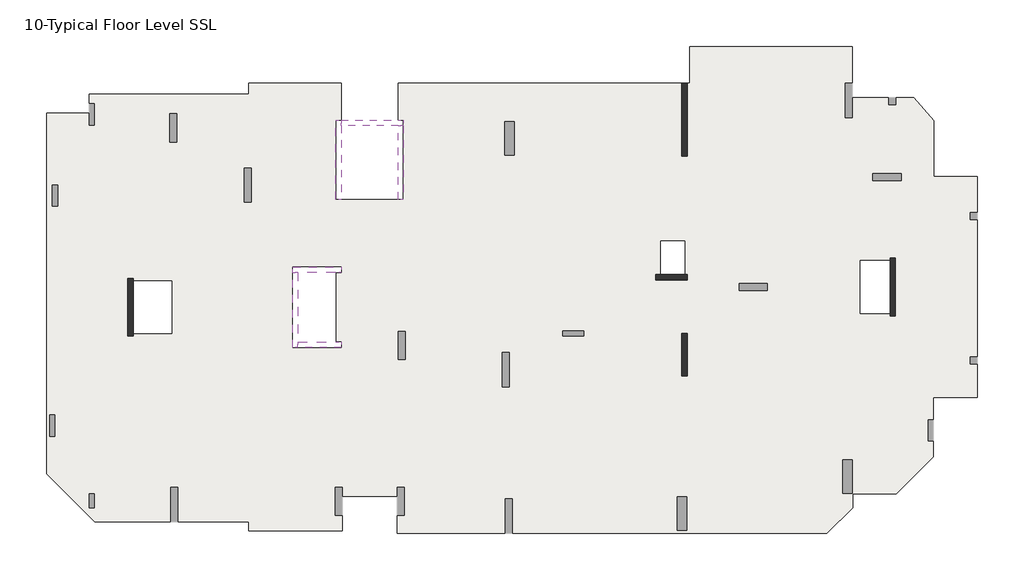
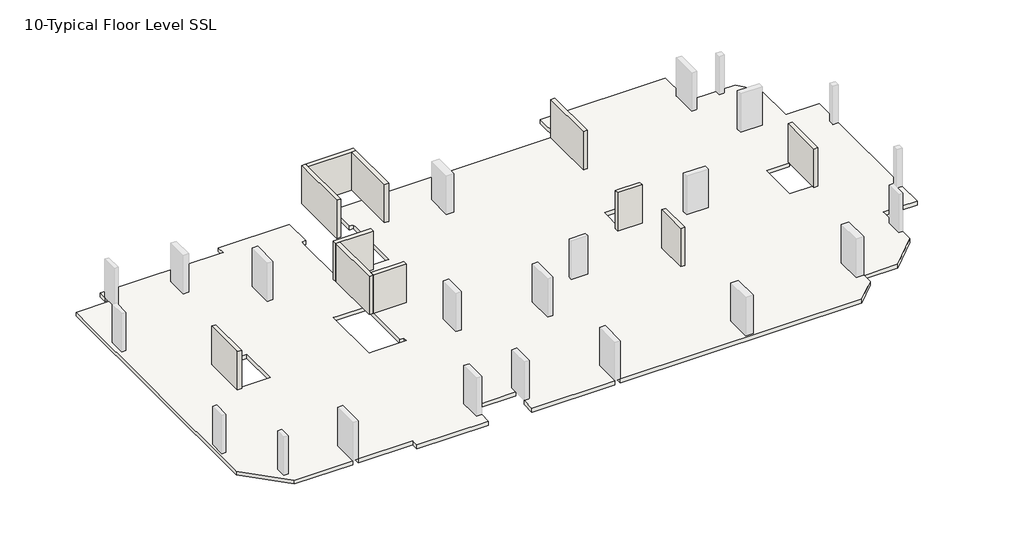
# One storey, part 1 of 2: 11 walls, 1 slab.
"""IFC4 building model written with IfcOpenShell, lengths in millimetres."""

from ifc_helpers import new_model, si_unit, origin, place, context, project, spatial, faceted_brep, element, save

model = new_model("IFC4")

# Units and contexts
model_context = context("Model", 3, world=origin())
ifc_project = project(units=[si_unit("LENGTHUNIT", "METRE", prefix="MILLI")], contexts=[model_context])

# Site, building, storey
site = spatial("IfcSite", under=ifc_project)
building = spatial("IfcBuilding", under=site)
storey = spatial("IfcBuildingStorey", under=building, Name="10-Typical Floor Level SSL", Elevation=24000.0)

# Slab
placement = place(None, origin())
element("IfcSlab", 1, ObjectType="Generic 300mm", at=placement, inside=storey, context=model_context, shape_type="Brep", body=[
    faceted_brep([(36192.0021644, 24072.000519, 23700.0), (36192.0021644, 26172.000519, 23700.0), (45446.0007483, 26172.000519, 23700.0), (45446.0007483, 24087.0, 23700.0), (45046.0007483, 24087.0, 23700.0), (45046.0007483, 22137.0, 23700.0), (45446.0007483, 22137.0, 23700.0), (45446.0007483, 23252.0000315, 23700.0), (47498.6337868, 23252.0000315, 23700.0), (47498.6337868, 22852.0, 23700.0), (47898.6337868, 22852.0, 23700.0), (47898.6337868, 23252.0000315, 23700.0), (48936.764334, 23252.0000315, 23700.0), (50076.0016214, 21956.8283806, 23700.0), (50076.0016214, 18780.0084406, 23700.0), (52549.9999998, 18780.0084406, 23700.0), (52549.9999998, 16712.0, 23700.0), (52149.9999998, 16712.0, 23700.0), (52149.9999998, 16312.0, 23700.0), (52549.9999998, 16312.0, 23700.0), (52549.9999998, 8504.0039609, 23700.0), (52149.9999998, 8504.0039609, 23700.0), (52149.9999998, 8104.0039609, 23700.0), (52549.9999998, 8104.0039609, 23700.0), (52549.9999998, 6204.0084406, 23700.0), (50046.0009271, 6204.0084406, 23700.0), (50046.0009271, 4931.9999929, 23700.0), (49746.0009271, 4931.9999929, 23700.0), (49746.0009271, 3731.9999929, 23700.0), (50046.0009271, 3731.9999929, 23700.0), (50046.0009271, 2810.5958657, 23700.0), (47943.4055804, 708.000519, 23700.0), (45456.0017287, 708.000519, 23700.0), (45456.0017287, -61.7051085, 23700.0), (43990.7023722, -1527.004465, 23700.0), (26113.9999998, -1527.004465, 23700.0), (26113.9999998, 422.995535, 23700.0), (25713.9999998, 422.995535, 23700.0), (25713.9999998, -1527.004465, 23700.0), (19569.9997488, -1527.004465, 23700.0), (19569.9997488, -512.0044652, 23700.0), (19969.9997488, -512.0044652, 23700.0), (19969.9997488, 1087.9955348, 23700.0), (19569.9997488, 1087.9955348, 23700.0), (19569.9997488, 564.000519, 23700.0), (16429.9999981, 564.000519, 23700.0), (16429.9999981, 1088.0, 23700.0), (16029.9999981, 1088.0, 23700.0), (16029.9999981, -512.0, 23700.0), (16429.9999981, -512.0, 23700.0), (16429.9999981, -1391.999481, 23700.0), (11136.0000923, -1391.999481, 23700.0), (11136.0000923, -866.9999847, 23700.0), (7082.0000416, -866.9999847, 23700.0), (7082.0000416, 1083.0000153, 23700.0), (6682.0000416, 1083.0000153, 23700.0), (6682.0000416, -866.9999847, 23700.0), (2364.4419097, -866.9999847, 23700.0), (-372.0, 1869.441925, 23700.0), (-372.0, 22380.0004589, 23700.0), (2052.0, 22380.0004589, 23700.0), (2052.0, 21708.0000656, 23700.0), (2352.0, 21708.0000656, 23700.0), (2352.0, 22908.0000656, 23700.0), (2052.0, 22908.0000656, 23700.0), (2052.0, 23472.000519, 23700.0), (11136.0000923, 23472.000519, 23700.0), (11136.0000923, 24072.000519, 23700.0), (16380.0000168, 24072.000519, 23700.0), (16380.0000168, 21972.0, 23700.0), (16079.9999997, 21972.0, 23700.0), (16079.9999997, 21672.0, 23700.0), (16079.9999997, 17468.0, 23700.0), (16379.9999997, 17468.0, 23700.0), (19619.9999997, 17468.0, 23700.0), (19919.9999997, 17468.0, 23700.0), (19919.9999997, 21672.0, 23700.0), (19919.9999997, 21972.0, 23700.0), (19619.9997365, 21972.0, 23700.0), (19619.9997365, 24072.000519, 23700.0), (35747.9999998, 24072.000519, 23700.0), (35747.9999998, 19932.0, 23700.0), (36047.9999998, 19932.0, 23700.0), (36047.9999998, 24072.000519, 23700.0), (16079.9999907, 9359.999998, 23700.0), (16079.9999907, 13320.0000002, 23700.0), (16380.0000168, 13320.0000002, 23700.0), (16380.0000168, 13620.0000002, 23700.0), (13919.9999907, 13620.0000002, 23700.0), (13619.9999907, 13620.0000002, 23700.0), (13619.9999907, 13320.0000002, 23700.0), (13619.9999907, 9359.999998, 23700.0), (13619.9999907, 9059.999998, 23700.0), (13919.9999907, 9059.999998, 23700.0), (16380.0000168, 9059.999998, 23700.0), (16380.0000168, 9359.999998, 23700.0), (4548.0000034, 9840.0000003, 23700.0), (6743.9999995, 9840.0000003, 23700.0), (6743.9999995, 12840.0000003, 23700.0), (4548.0000034, 12840.0000003, 23700.0), (4548.0000025, 12984.0000001, 23700.0), (4248.0000025, 12984.0000001, 23700.0), (4248.0000025, 9696.0, 23700.0), (4548.0000025, 9696.0, 23700.0), (47580.0014798, 13992.0079177, 23700.0), (45900.001729, 13992.0079177, 23700.0), (45900.001729, 10992.0079181, 23700.0), (47580.0014798, 10992.0079181, 23700.0), (47580.0014811, 10848.0079202, 23700.0), (47880.0014811, 10848.0079202, 23700.0), (47880.0014811, 14136.0000002, 23700.0), (47580.0014811, 14136.0000002, 23700.0), (35904.002157, 15108.0000083, 23700.0), (34548.0015145, 15108.0000083, 23700.0), (34548.0015145, 13199.9999992, 23700.0), (34248.0015201, 13199.9999992, 23700.0), (34248.0015201, 12899.9999992, 23700.0), (36048.0015201, 12899.9999992, 23700.0), (36048.0015201, 13199.9999992, 23700.0), (35904.002157, 13199.9999992, 23700.0), (257.9999999, 17088.0, 23700.0), (257.9999999, 18288.0, 23700.0), (-42.0000001, 18288.0, 23700.0), (-42.0000001, 17088.0, 23700.0), (108.001803, 4001.9999858, 23700.0), (108.001803, 5201.9999858, 23700.0), (-191.998197, 5201.9999858, 23700.0), (-191.998197, 4001.9999858, 23700.0), (30175.9999998, 9996.0000019, 23700.0), (28975.9999998, 9996.0000019, 23700.0), (28975.9999998, 9696.0000019, 23700.0), (30175.9999998, 9696.0000019, 23700.0), (7021.9999999, 20740.0000078, 23700.0), (7021.9999999, 22340.0000078, 23700.0), (6621.9999999, 22340.0000078, 23700.0), (6621.9999999, 20740.0000078, 23700.0), (48205.9993605, 18950.0, 23700.0), (46605.9993605, 18950.0, 23700.0), (46605.9993605, 18550.0, 23700.0), (48205.9993605, 18550.0, 23700.0), (20030.000009, 8355.9999979, 23700.0), (20030.000009, 9955.9999979, 23700.0), (19630.000009, 9955.9999979, 23700.0), (19630.000009, 8355.9999979, 23700.0), (11270.0000427, 17312.9999996, 23700.0), (11270.0000427, 19262.9999996, 23700.0), (10870.0000427, 19262.9999996, 23700.0), (10870.0000427, 17312.9999996, 23700.0), (40598.0014887, 12692.0079212, 23700.0), (38998.0014887, 12692.0079212, 23700.0), (38998.0014887, 12292.0079212, 23700.0), (40598.0014887, 12292.0079212, 23700.0), (2352.0, -72.0, 23700.0), (2352.0, 728.0, 23700.0), (2052.0, 728.0, 23700.0), (2052.0, -72.0, 23700.0), (25934.0000455, 6801.0001824, 23700.0), (25934.0000455, 8751.0001824, 23700.0), (25534.0000455, 8751.0001824, 23700.0), (25534.0000455, 6801.0001824, 23700.0), (36035.9999998, -1351.9992017, 23700.0), (36035.9999998, 548.0007983, 23700.0), (35485.9999998, 548.0007983, 23700.0), (35485.9999998, -1351.9992017, 23700.0), (45443.9999998, 748.0, 23700.0), (45443.9999998, 2648.0, 23700.0), (44893.9999998, 2648.0, 23700.0), (44893.9999998, 748.0, 23700.0), (26218.9999998, 20000.0, 23700.0), (26218.9999998, 21900.0, 23700.0), (25668.9999998, 21900.0, 23700.0), (25668.9999998, 20000.0, 23700.0), (35748.0054035, 9840.0000002, 23700.0), (35748.0054035, 7428.0000762, 23700.0), (36048.0054035, 7428.0000762, 23700.0), (36048.0054035, 9840.0000002, 23700.0), (36192.0021644, 26172.000519, 24000.0), (36192.0021644, 24072.000519, 24000.0), (36047.9999998, 24072.000519, 24000.0), (36047.9999998, 19932.0, 24000.0), (35747.9999998, 19932.0, 24000.0), (35747.9999998, 24072.000519, 24000.0), (19619.9997365, 24072.000519, 24000.0), (19619.9997365, 21972.0, 24000.0), (19919.9999997, 21972.0, 24000.0), (19919.9999997, 21672.0, 24000.0), (19919.9999997, 17468.0, 24000.0), (19619.9999997, 17468.0, 24000.0), (16379.9999997, 17468.0, 24000.0), (16079.9999997, 17468.0, 24000.0), (16079.9999997, 21672.0, 24000.0), (16079.9999997, 21972.0, 24000.0), (16380.0000168, 21972.0, 24000.0), (16380.0000168, 24072.000519, 24000.0), (11136.0000923, 24072.000519, 24000.0), (11136.0000923, 23472.000519, 24000.0), (2052.0, 23472.000519, 24000.0), (2052.0, 22908.0000656, 24000.0), (2352.0, 22908.0000656, 24000.0), (2352.0, 21708.0000656, 24000.0), (2052.0, 21708.0000656, 24000.0), (2052.0, 22380.0004589, 24000.0), (-372.0, 22380.0004589, 24000.0), (-372.0, 1869.441925, 24000.0), (2364.4419097, -866.9999847, 24000.0), (6682.0000416, -866.9999847, 24000.0), (6682.0000416, 1083.0000153, 24000.0), (7082.0000416, 1083.0000153, 24000.0), (7082.0000416, -866.9999847, 24000.0), (11136.0000923, -866.9999847, 24000.0), (11136.0000923, -1391.999481, 24000.0), (16429.9999981, -1391.999481, 24000.0), (16429.9999981, -512.0, 24000.0), (16029.9999981, -512.0, 24000.0), (16029.9999981, 1088.0, 24000.0), (16429.9999981, 1088.0, 24000.0), (16429.9999981, 564.000519, 24000.0), (19569.9997488, 564.000519, 24000.0), (19569.9997488, 1087.9955348, 24000.0), (19969.9997488, 1087.9955348, 24000.0), (19969.9997488, -512.0044652, 24000.0), (19569.9997488, -512.0044652, 24000.0), (19569.9997488, -1527.004465, 24000.0), (25713.9999998, -1527.004465, 24000.0), (25713.9999998, 422.995535, 24000.0), (26113.9999998, 422.995535, 24000.0), (26113.9999998, -1527.004465, 24000.0), (43990.7023722, -1527.004465, 24000.0), (45456.0017287, -61.7051085, 24000.0), (45456.0017287, 708.000519, 24000.0), (47943.4055804, 708.000519, 24000.0), (50046.0009271, 2810.5958657, 24000.0), (50046.0009271, 3731.9999929, 24000.0), (49746.0009271, 3731.9999929, 24000.0), (49746.0009271, 4931.9999929, 24000.0), (50046.0009271, 4931.9999929, 24000.0), (50046.0009271, 6204.0084406, 24000.0), (52549.9999998, 6204.0084406, 24000.0), (52549.9999998, 8104.0039609, 24000.0), (52149.9999998, 8104.0039609, 24000.0), (52149.9999998, 8504.0039609, 24000.0), (52549.9999998, 8504.0039609, 24000.0), (52549.9999998, 16312.0, 24000.0), (52149.9999998, 16312.0, 24000.0), (52149.9999998, 16712.0, 24000.0), (52549.9999998, 16712.0, 24000.0), (52549.9999998, 18780.0084406, 24000.0), (50076.0016214, 18780.0084406, 24000.0), (50076.0016214, 21956.8283806, 24000.0), (48936.764334, 23252.0000315, 24000.0), (47898.6337868, 23252.0000315, 24000.0), (47898.6337868, 22852.0, 24000.0), (47498.6337868, 22852.0, 24000.0), (47498.6337868, 23252.0000315, 24000.0), (45446.0006898, 23252.0000315, 24000.0), (45446.0007483, 22137.0, 24000.0), (45046.0007483, 22137.0, 24000.0), (45046.0007483, 24087.0, 24000.0), (45446.0007483, 24087.0, 24000.0), (45446.0007483, 26172.000519, 24000.0), (16079.9999907, 13320.0000002, 24000.0), (16079.9999907, 9359.999998, 24000.0), (16380.0000168, 9359.999998, 24000.0), (16380.0000168, 9059.999998, 24000.0), (13919.9999907, 9059.999998, 24000.0), (13619.9999907, 9059.999998, 24000.0), (13619.9999907, 9359.999998, 24000.0), (13619.9999907, 13320.0000002, 24000.0), (13619.9999907, 13620.0000002, 24000.0), (13919.9999907, 13620.0000002, 24000.0), (16380.0000168, 13620.0000002, 24000.0), (16380.0000168, 13320.0000002, 24000.0), (6743.9999995, 9840.0000003, 24000.0), (4548.0000034, 9840.0000003, 24000.0), (4548.0000025, 9696.0, 24000.0), (4248.0000025, 9696.0, 24000.0), (4248.0000025, 12984.0000001, 24000.0), (4548.0000025, 12984.0000001, 24000.0), (4548.0000025, 12840.0000003, 24000.0), (6743.9999995, 12840.0000003, 24000.0), (45900.001729, 13992.0079177, 24000.0), (47580.0014798, 13992.0079177, 24000.0), (47580.0014811, 14136.0000002, 24000.0), (47880.0014811, 14136.0000002, 24000.0), (47880.0014811, 10848.0079202, 24000.0), (47580.0014811, 10848.0079202, 24000.0), (47580.0014811, 10992.0079181, 24000.0), (45900.001729, 10992.0079181, 24000.0), (34548.0015145, 15108.0000083, 24000.0), (35904.002157, 15108.0000083, 24000.0), (35904.002157, 13199.9999992, 24000.0), (36048.0015201, 13199.9999992, 24000.0), (36048.0015201, 12899.9999992, 24000.0), (34248.0015201, 12899.9999992, 24000.0), (34248.0015201, 13199.9999992, 24000.0), (34548.0015145, 13199.9999992, 24000.0), (257.9999999, 18288.0, 24000.0), (257.9999999, 17088.0, 24000.0), (-42.0000001, 17088.0, 24000.0), (-42.0000001, 18288.0, 24000.0), (108.001803, 5201.9999858, 24000.0), (108.001803, 4001.9999858, 24000.0), (-191.998197, 4001.9999858, 24000.0), (-191.998197, 5201.9999858, 24000.0), (28975.9999998, 9996.0000019, 24000.0), (30175.9999998, 9996.0000019, 24000.0), (30175.9999998, 9696.0000019, 24000.0), (28975.9999998, 9696.0000019, 24000.0), (7021.9999999, 22340.0000078, 24000.0), (7021.9999999, 20740.0000078, 24000.0), (6621.9999999, 20740.0000078, 24000.0), (6621.9999999, 22340.0000078, 24000.0), (46605.9993605, 18950.0, 24000.0), (48205.9993605, 18950.0, 24000.0), (48205.9993605, 18550.0, 24000.0), (46605.9993605, 18550.0, 24000.0), (20030.000009, 9955.9999979, 24000.0), (20030.000009, 8355.9999979, 24000.0), (19630.000009, 8355.9999979, 24000.0), (19630.000009, 9955.9999979, 24000.0), (11270.0000427, 19262.9999996, 24000.0), (11270.0000427, 17312.9999996, 24000.0), (10870.0000427, 17312.9999996, 24000.0), (10870.0000427, 19262.9999996, 24000.0), (38998.0014887, 12692.0079212, 24000.0), (40598.0014887, 12692.0079212, 24000.0), (40598.0014887, 12292.0079212, 24000.0), (38998.0014887, 12292.0079212, 24000.0), (2352.0, 728.0, 24000.0), (2352.0, -72.0, 24000.0), (2052.0, -72.0, 24000.0), (2052.0, 728.0, 24000.0), (25934.0000455, 8751.0001824, 24000.0), (25934.0000455, 6801.0001824, 24000.0), (25534.0000455, 6801.0001824, 24000.0), (25534.0000455, 8751.0001824, 24000.0), (36035.9999998, 548.0007983, 24000.0), (36035.9999998, -1351.9992017, 24000.0), (35485.9999998, -1351.9992017, 24000.0), (35485.9999998, 548.0007983, 24000.0), (45443.9999998, 2648.0, 24000.0), (45443.9999998, 748.0, 24000.0), (44893.9999998, 748.0, 24000.0), (44893.9999998, 2648.0, 24000.0), (26218.9999998, 21900.0, 24000.0), (26218.9999998, 20000.0, 24000.0), (25668.9999998, 20000.0, 24000.0), (25668.9999998, 21900.0, 24000.0), (35748.0054035, 7428.0000762, 24000.0), (35748.0054035, 9840.0000002, 24000.0), (36048.0054035, 9840.0000002, 24000.0), (36048.0054035, 7428.0000762, 24000.0)], [[[0, 1, 2, 3, 4, 5, 6, 7, 8, 9, 10, 11, 12, 13, 14, 15, 16, 17, 18, 19, 20, 21, 22, 23, 24, 25, 26, 27, 28, 29, 30, 31, 32, 33, 34, 35, 36, 37, 38, 39, 40, 41, 42, 43, 44, 45, 46, 47, 48, 49, 50, 51, 52, 53, 54, 55, 56, 57, 58, 59, 60, 61, 62, 63, 64, 65, 66, 67, 68, 69, 70, 71, 72, 73, 74, 75, 76, 77, 78, 79, 80, 81, 82, 83], [84, 85, 86, 87, 88, 89, 90, 91, 92, 93, 94, 95], [96, 97, 98, 99, 100, 101, 102, 103], [104, 105, 106, 107, 108, 109, 110, 111], [112, 113, 114, 115, 116, 117, 118, 119], [120, 121, 122, 123], [124, 125, 126, 127], [128, 129, 130, 131], [132, 133, 134, 135], [136, 137, 138, 139], [140, 141, 142, 143], [144, 145, 146, 147], [148, 149, 150, 151], [152, 153, 154, 155], [156, 157, 158, 159], [160, 161, 162, 163], [164, 165, 166, 167], [168, 169, 170, 171], [172, 173, 174, 175]], [[176, 177, 178, 179, 180, 181, 182, 183, 184, 185, 186, 187, 188, 189, 190, 191, 192, 193, 194, 195, 196, 197, 198, 199, 200, 201, 202, 203, 204, 205, 206, 207, 208, 209, 210, 211, 212, 213, 214, 215, 216, 217, 218, 219, 220, 221, 222, 223, 224, 225, 226, 227, 228, 229, 230, 231, 232, 233, 234, 235, 236, 237, 238, 239, 240, 241, 242, 243, 244, 245, 246, 247, 248, 249, 250, 251, 252, 253, 254, 255, 256, 257, 258, 259], [260, 261, 262, 263, 264, 265, 266, 267, 268, 269, 270, 271], [272, 273, 274, 275, 276, 277, 278, 279], [280, 281, 282, 283, 284, 285, 286, 287], [288, 289, 290, 291, 292, 293, 294, 295], [296, 297, 298, 299], [300, 301, 302, 303], [304, 305, 306, 307], [308, 309, 310, 311], [312, 313, 314, 315], [316, 317, 318, 319], [320, 321, 322, 323], [324, 325, 326, 327], [328, 329, 330, 331], [332, 333, 334, 335], [336, 337, 338, 339], [340, 341, 342, 343], [344, 345, 346, 347], [348, 349, 350, 351]], [[68, 193, 192, 69]], [[182, 79, 78, 183]], [[79, 182, 181, 80]], [[177, 0, 83, 178]], [[1, 0, 177, 176]], [[2, 1, 176, 259]], [[3, 2, 259, 258]], [[249, 12, 11, 250]], [[7, 254, 253, 8]], [[13, 12, 249, 248]], [[14, 13, 248, 247]], [[15, 14, 247, 246]], [[15, 246, 245, 16]], [[237, 24, 23, 238]], [[19, 242, 241, 20]], [[25, 24, 237, 236]], [[25, 236, 235, 26]], [[231, 30, 29, 232]], [[32, 31, 230, 229]], [[33, 32, 229, 228]], [[34, 33, 228, 227]], [[34, 227, 226, 35]], [[222, 39, 38, 223]], [[39, 222, 221, 40]], [[45, 44, 217, 216]], [[211, 50, 49, 212]], [[51, 50, 211, 210]], [[52, 51, 210, 209]], [[52, 209, 208, 53]], [[204, 57, 56, 205]], [[58, 57, 204, 203]], [[59, 58, 203, 202]], [[60, 59, 202, 201]], [[196, 65, 64, 197]], [[66, 65, 196, 195]], [[67, 66, 195, 194]], [[68, 67, 194, 193]], [[31, 30, 231, 230]], [[85, 84, 261, 260]], [[72, 189, 188, 187, 186, 75, 74, 73]], [[272, 97, 96, 273]], [[97, 272, 279, 98]], [[98, 279, 278, 99]], [[280, 105, 104, 281]], [[105, 280, 287, 106]], [[106, 287, 286, 107]], [[112, 289, 288, 113]], [[113, 288, 295, 114]], [[289, 112, 119, 290]], [[62, 199, 198, 63]], [[199, 62, 61, 200]], [[200, 61, 60, 201]], [[63, 198, 197, 64]], [[120, 297, 296, 121]], [[297, 120, 123, 298]], [[298, 123, 122, 299]], [[299, 122, 121, 296]], [[124, 301, 300, 125]], [[301, 124, 127, 302]], [[302, 127, 126, 303]], [[303, 126, 125, 300]], [[28, 233, 232, 29]], [[233, 28, 27, 234]], [[234, 27, 26, 235]], [[128, 305, 304, 129]], [[305, 128, 131, 306]], [[306, 131, 130, 307]], [[307, 130, 129, 304]], [[132, 309, 308, 133]], [[309, 132, 135, 310]], [[310, 135, 134, 311]], [[311, 134, 133, 308]], [[41, 220, 219, 42]], [[220, 41, 40, 221]], [[43, 218, 217, 44]], [[218, 43, 42, 219]], [[136, 313, 312, 137]], [[313, 136, 139, 314]], [[314, 139, 138, 315]], [[315, 138, 137, 312]], [[140, 317, 316, 141]], [[317, 140, 143, 318]], [[318, 143, 142, 319]], [[319, 142, 141, 316]], [[215, 46, 45, 216]], [[48, 213, 212, 49]], [[213, 48, 47, 214]], [[214, 47, 46, 215]], [[144, 321, 320, 145]], [[321, 144, 147, 322]], [[322, 147, 146, 323]], [[323, 146, 145, 320]], [[207, 54, 53, 208]], [[55, 206, 205, 56]], [[206, 55, 54, 207]], [[225, 36, 35, 226]], [[37, 224, 223, 38]], [[224, 37, 36, 225]], [[6, 255, 254, 7]], [[255, 6, 5, 256]], [[256, 5, 4, 257]], [[257, 4, 3, 258]], [[148, 325, 324, 149]], [[325, 148, 151, 326]], [[326, 151, 150, 327]], [[327, 150, 149, 324]], [[152, 329, 328, 153]], [[329, 152, 155, 330]], [[330, 155, 154, 331]], [[331, 154, 153, 328]], [[156, 333, 332, 157]], [[333, 156, 159, 334]], [[334, 159, 158, 335]], [[335, 158, 157, 332]], [[160, 337, 336, 161]], [[337, 160, 163, 338]], [[338, 163, 162, 339]], [[339, 162, 161, 336]], [[164, 341, 340, 165]], [[341, 164, 167, 342]], [[342, 167, 166, 343]], [[343, 166, 165, 340]], [[168, 345, 344, 169]], [[345, 168, 171, 346]], [[346, 171, 170, 347]], [[347, 170, 169, 344]], [[70, 191, 190, 189, 72, 71]], [[191, 70, 69, 192]], [[77, 184, 183, 78]], [[184, 77, 76, 75, 186, 185]], [[271, 86, 85, 260]], [[87, 270, 269, 268, 89, 88]], [[86, 271, 270, 87]], [[89, 268, 267, 266, 265, 92, 91, 90]], [[92, 265, 264, 263, 94, 93]], [[95, 262, 261, 84]], [[262, 95, 94, 263]], [[277, 100, 99, 278]], [[103, 274, 273, 96]], [[101, 276, 275, 102]], [[100, 277, 276, 101]], [[274, 103, 102, 275]], [[116, 293, 292, 117]], [[118, 291, 290, 119]], [[294, 115, 114, 295]], [[117, 292, 291, 118]], [[293, 116, 115, 294]], [[172, 349, 348, 173]], [[174, 351, 350, 175]], [[173, 348, 351, 174]], [[349, 172, 175, 350]], [[285, 108, 107, 286]], [[111, 282, 281, 104]], [[109, 284, 283, 110]], [[108, 285, 284, 109]], [[282, 111, 110, 283]], [[82, 179, 178, 83]], [[180, 81, 80, 181]], [[179, 82, 81, 180]], [[18, 243, 242, 19]], [[243, 18, 17, 244]], [[244, 17, 16, 245]], [[10, 251, 250, 11]], [[251, 10, 9, 252]], [[252, 9, 8, 253]], [[22, 239, 238, 23]], [[239, 22, 21, 240]], [[240, 21, 20, 241]]]),
])

# Walls
element("IfcWall", 2, ObjectType="Shear Walls 300mm", at=placement, inside=storey, context=model_context, shape_type="Brep", body=[
    faceted_brep([(4548.0000025, 9696.0, 24000.0), (4548.0000025, 12984.0000001, 24000.0), (4548.0000025, 12984.0000001, 26700.0), (4548.0000025, 12984.0000001, 27000.0), (4548.0000025, 12840.0000003, 27000.0), (4548.0000025, 9840.0000003, 27000.0), (4548.0000025, 9696.0, 27000.0), (4548.0000025, 9696.0, 26700.0), (4248.0000025, 9696.0, 24000.0), (4248.0000025, 9696.0, 26700.0), (4248.0000025, 9696.0, 27000.0), (4248.0000025, 12984.0000001, 27000.0), (4248.0000025, 12984.0000001, 26700.0), (4248.0000025, 12984.0000001, 24000.0)], [[[0, 1, 2, 3, 4, 5, 6, 7]], [[8, 9, 10, 11, 12, 13]], [[1, 0, 8, 13]], [[3, 2, 1, 13, 12, 11]], [[6, 5, 4, 3, 11, 10]], [[0, 7, 6, 10, 9, 8]]]),
])
element("IfcWall", 3, ObjectType="Shear Walls 300mm", at=placement, inside=storey, context=model_context, shape_type="Brep", body=[
    faceted_brep([(34248.0015201, 12899.9999992, 24000.0), (36048.0015201, 12899.9999992, 24000.0), (36048.0015201, 12899.9999992, 26700.0), (36048.0015201, 12899.9999992, 27000.0), (34248.0015201, 12899.9999992, 27000.0), (34248.0015201, 12899.9999992, 26700.0), (34248.0015201, 13199.9999992, 24000.0), (34248.0015201, 13199.9999992, 26700.0), (34248.0015201, 13199.9999992, 27000.0), (34548.0015145, 13199.9999992, 27000.0), (35904.002157, 13199.9999992, 27000.0), (36048.0015201, 13199.9999992, 27000.0), (36048.0015201, 13199.9999992, 26700.0), (36048.0015201, 13199.9999992, 24000.0)], [[[0, 1, 2, 3, 4, 5]], [[6, 7, 8, 9, 10, 11, 12, 13]], [[1, 0, 6, 13]], [[3, 2, 1, 13, 12, 11]], [[4, 3, 11, 10, 9, 8]], [[0, 5, 4, 8, 7, 6]]]),
])
element("IfcWall", 4, ObjectType="Shear Walls 300mm", at=placement, inside=storey, context=model_context, shape_type="Brep", body=[
    faceted_brep([(35748.0054035, 9840.0000002, 24000.0), (35748.0054035, 7428.0000762, 24000.0), (35748.0054035, 7428.0000762, 26700.0), (35748.0054035, 7428.0000762, 27000.0), (35748.0054035, 9840.0000002, 27000.0), (35748.0054035, 9840.0000002, 26700.0), (36048.0054035, 9840.0000002, 24000.0), (36048.0054035, 9840.0000002, 26700.0), (36048.0054035, 9840.0000002, 27000.0), (36048.0054035, 7428.0000762, 27000.0), (36048.0054035, 7428.0000762, 26700.0), (36048.0054035, 7428.0000762, 24000.0)], [[[0, 1, 2, 3, 4, 5]], [[6, 7, 8, 9, 10, 11]], [[1, 0, 6, 11]], [[3, 2, 1, 11, 10, 9]], [[4, 3, 9, 8]], [[0, 5, 4, 8, 7, 6]]]),
])
element("IfcWall", 5, ObjectType="Shear Walls 300mm", at=placement, inside=storey, context=model_context, shape_type="Brep", body=[
    faceted_brep([(47580.0014811, 14136.0000002, 24000.0), (47580.0014811, 10848.0079202, 24000.0), (47580.0014811, 10848.0079202, 26700.0), (47580.0014811, 10848.0079202, 27000.0), (47580.0014811, 10992.0079181, 27000.0), (47580.0014811, 13992.0079177, 27000.0), (47580.0014811, 14136.0000002, 27000.0), (47580.0014811, 14136.0000002, 26700.0), (47880.0014811, 14136.0000002, 24000.0), (47880.0014811, 14136.0000002, 26700.0), (47880.0014811, 14136.0000002, 27000.0), (47880.0014811, 10848.0079202, 27000.0), (47880.0014811, 10848.0079202, 26700.0), (47880.0014811, 10848.0079202, 24000.0)], [[[0, 1, 2, 3, 4, 5, 6, 7]], [[8, 9, 10, 11, 12, 13]], [[1, 0, 8, 13]], [[3, 2, 1, 13, 12, 11]], [[6, 5, 4, 3, 11, 10]], [[0, 7, 6, 10, 9, 8]]]),
])
element("IfcWall", 6, ObjectType="Shear Walls 300mm", at=placement, inside=storey, context=model_context, shape_type="Brep", body=[
    faceted_brep([(36047.9999998, 19932.0, 24000.0), (36047.9999998, 24072.0078999, 24000.0), (36047.9999998, 24072.0078999, 27000.0), (36047.9999998, 19932.0, 27000.0), (36047.9999998, 19932.0, 26700.0), (35747.9999998, 19932.0, 24000.0), (35747.9999998, 19932.0, 26700.0), (35747.9999998, 19932.0, 27000.0), (35747.9999998, 24072.0078999, 27000.0), (35747.9999998, 24072.0078999, 24000.0)], [[[0, 1, 2, 3, 4]], [[5, 6, 7, 8, 9]], [[1, 0, 5, 9]], [[2, 1, 9, 8]], [[3, 2, 8, 7]], [[0, 4, 3, 7, 6, 5]]]),
])
element("IfcWall", 7, ObjectType="Shear Walls 300mm", at=placement, inside=storey, context=model_context, shape_type="Brep", body=[
    faceted_brep([(16379.9999997, 21972.0, 30000.0), (16379.9999997, 21672.0, 30000.0), (16379.9999997, 17468.0, 30000.0), (16379.9999997, 17468.0, 27000.0), (16379.9999997, 21672.0, 27000.0), (16379.9999997, 21972.0, 27000.0), (16079.9999997, 17468.0, 30000.0), (16079.9999997, 21972.0, 30000.0), (16079.9999997, 21972.0, 29700.0), (16079.9999997, 21972.0, 27000.0), (16079.9999997, 17468.0, 27000.0), (16079.9999997, 17468.0, 29700.0)], [[[0, 1, 2, 3, 4, 5]], [[6, 7, 8, 9, 10, 11]], [[2, 1, 0, 7, 6]], [[2, 6, 11, 10, 3]], [[3, 10, 9, 5, 4]], [[0, 5, 9, 8, 7]]]),
])
element("IfcWall", 8, ObjectType="Shear Walls 300mm", at=placement, inside=storey, context=model_context, shape_type="Brep", body=[
    faceted_brep([(16379.9999997, 21972.0, 30000.0), (19619.9997365, 21972.0, 30000.0), (19919.9999997, 21972.0, 30000.0), (19919.9999997, 21972.0, 29700.0), (19919.9999997, 21972.0, 27000.0), (16379.9999997, 21972.0, 27000.0), (19919.9999997, 21672.0, 30000.0), (19619.9999997, 21672.0, 30000.0), (16379.9999997, 21672.0, 30000.0), (16379.9999997, 21672.0, 27000.0), (19619.9999997, 21672.0, 27000.0), (19919.9999997, 21672.0, 27000.0)], [[[0, 1, 2, 3, 4, 5]], [[6, 7, 8, 9, 10, 11]], [[2, 1, 0, 8, 7, 6]], [[8, 0, 5, 9]], [[9, 5, 4, 11, 10]], [[4, 3, 2, 6, 11]]]),
])
element("IfcWall", 9, ObjectType="Shear Walls 300mm", at=placement, inside=storey, context=model_context, shape_type="Brep", body=[
    faceted_brep([(19919.9999997, 21672.0, 30000.0), (19919.9999997, 17468.0, 30000.0), (19919.9999997, 17468.0, 29700.0), (19919.9999997, 17468.0, 27000.0), (19919.9999997, 21672.0, 27000.0), (19619.9999997, 17468.0, 30000.0), (19619.9999997, 21672.0, 30000.0), (19619.9999997, 21672.0, 27000.0), (19619.9999997, 17468.0, 27000.0)], [[[0, 1, 2, 3, 4]], [[5, 6, 7, 8]], [[1, 0, 6, 5]], [[1, 5, 8, 3, 2]], [[6, 0, 4, 7]], [[4, 3, 8, 7]]]),
])
element("IfcWall", 10, ObjectType="Shear Walls 300mm", at=placement, inside=storey, context=model_context, shape_type="Brep", body=[
    faceted_brep([(16380.0000168, 13320.0000002, 30000.0), (16079.9999907, 13320.0000002, 30000.0), (13919.9999907, 13320.0000002, 30000.0), (13619.9999907, 13320.0000002, 30000.0), (13619.9999907, 13320.0000002, 27000.0), (13919.9999907, 13320.0000002, 27000.0), (16380.0000168, 13320.0000002, 27000.0), (16380.0000168, 13320.0000002, 29700.0), (13619.9999907, 13620.0000002, 30000.0), (16380.0000168, 13620.0000002, 30000.0), (16380.0000168, 13620.0000002, 29700.0), (16380.0000168, 13620.0000002, 27000.0), (13619.9999907, 13620.0000002, 27000.0), (13619.9999907, 13620.0000002, 29700.0)], [[[0, 1, 2, 3, 4, 5, 6, 7]], [[8, 9, 10, 11, 12, 13]], [[9, 0, 7, 6, 11, 10]], [[3, 2, 1, 0, 9, 8]], [[11, 6, 5, 4, 12]], [[4, 3, 8, 13, 12]]]),
])
element("IfcWall", 11, ObjectType="Shear Walls 300mm", at=placement, inside=storey, context=model_context, shape_type="Brep", body=[
    faceted_brep([(13919.9999907, 13320.0000002, 30000.0), (13919.9999907, 9359.999998, 30000.0), (13919.9999907, 9059.999998, 30000.0), (13919.9999907, 9059.999998, 27000.0), (13919.9999907, 9359.999998, 27000.0), (13919.9999907, 13320.0000002, 27000.0), (13619.9999907, 9059.999998, 30000.0), (13619.9999907, 13320.0000002, 30000.0), (13619.9999907, 13320.0000002, 27000.0), (13619.9999907, 9059.999998, 27000.0), (13619.9999907, 9059.999998, 29700.0)], [[[0, 1, 2, 3, 4, 5]], [[6, 7, 8, 9, 10]], [[2, 1, 0, 7, 6]], [[7, 0, 5, 8]], [[8, 5, 4, 3, 9]], [[3, 2, 6, 10, 9]]]),
])
element("IfcWall", 12, ObjectType="Shear Walls 300mm", at=placement, inside=storey, context=model_context, shape_type="Brep", body=[
    faceted_brep([(13919.9999907, 9359.999998, 30000.0), (16079.9999907, 9359.999998, 30000.0), (16380.0000168, 9359.999998, 30000.0), (16380.0000168, 9359.999998, 29700.0), (16380.0000168, 9359.999998, 27000.0), (13919.9999907, 9359.999998, 27000.0), (16380.0000168, 9059.999998, 30000.0), (13919.9999907, 9059.999998, 30000.0), (13919.9999907, 9059.999998, 27000.0), (16380.0000168, 9059.999998, 27000.0), (16380.0000168, 9059.999998, 29700.0)], [[[0, 1, 2, 3, 4, 5]], [[6, 7, 8, 9, 10]], [[2, 1, 0, 7, 6]], [[2, 6, 10, 9, 4, 3]], [[7, 0, 5, 8]], [[5, 4, 9, 8]]]),
])

save(model, "model.ifc")

# Revit data of these elements
# Type "Generic 300mm"
#   Function = 0
#   Layers, outside or top first: 300 mm "Concrete-RC" (function 1)
# Type "Shear Walls 300mm"
#   Layers, outside or top first: 300 mm "Concrete-RC" (function 1)
# Element 1 (IfcSlab, "Generic 300mm")
#   Height Offset From Level = 0 mm
#   built-in parameter 1001954 = 1
#   Phase Created = New Construction
#   Materials on its faces: "Concrete-RC"
# Elements 2, 3, 4, 5, 6 (IfcWall, "Shear Walls 300mm")
#   Top Offset = 0 mm
#   Base Offset = 0 mm
#   wall height = 3000 mm
#   Phase Created = New Construction
#   Base Constraint = 10-Typical Floor Level SSL
#   Top Constraint = 11-Typical Floor Level SSL
#   Materials on its faces: "Concrete-RC"
# Elements 7, 8, 9, 10, 11, 12 (IfcWall, "Shear Walls 300mm")
#   Top Offset = 0 mm
#   Base Offset = 0 mm
#   wall height = 6000 mm
#   Phase Created = New Construction
#   Base Constraint = 10-Typical Floor Level SSL
#   Top Constraint = 12-Typical Floor Level SSL
#   Materials on its faces: "Concrete-RC"
# Materials
#   "Concrete-RC": class "Concrete", colour RGB 128 128 128, transparency 0, Description = "High strength concrete", Cost = 0
